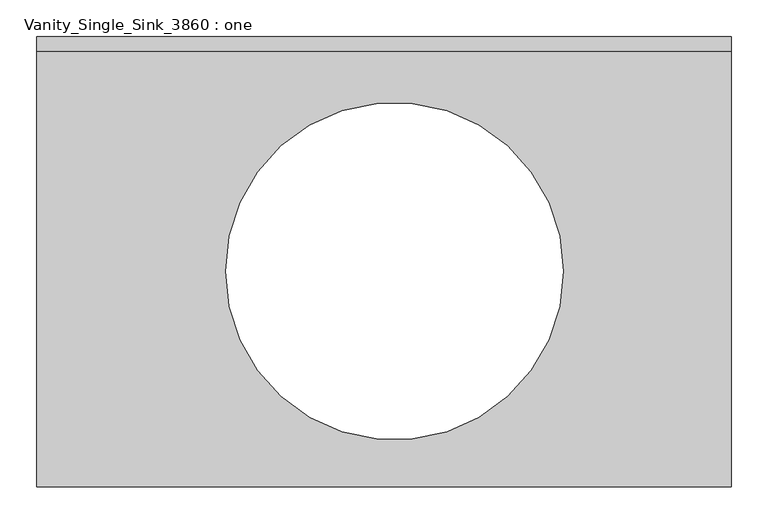
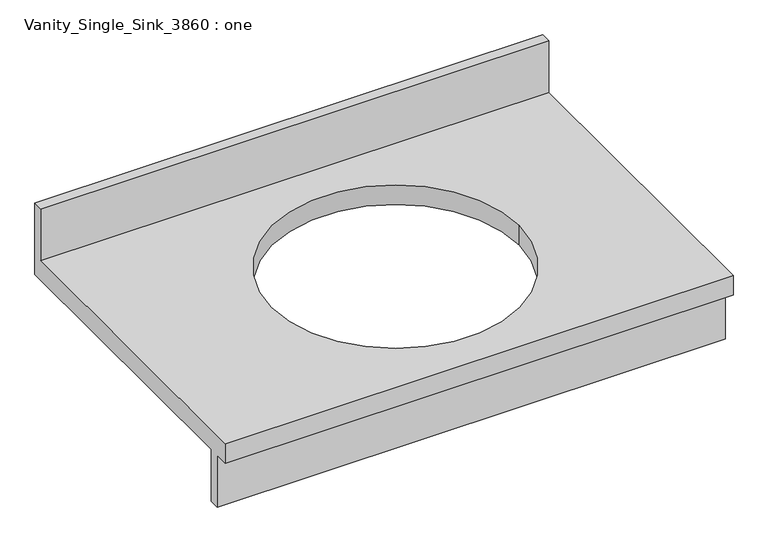
"""IFC4 building model written with IfcOpenShell, lengths in millimetres: furniture geometry, Vanity_Single_Sink_3860 : one."""

import ifcopenshell
import ifcopenshell.guid

model = None  # the IFC model being written
_history = None  # IfcOwnerHistory: only IFC2X3 demands one
_inside = {}  # id of a spatial element -> (the spatial element, [elements in it])
_under = {}  # id of a project, library or spatial element -> (it, [spatial elements below it])
_declared = {}  # id of a project -> (the project, [libraries it declares])
_typed = {}  # id of a type object -> (the type object, [elements of that type])
_made_of = {}  # id of a material, layer set ... -> (it, [elements and type objects made of it])


def new_model(schema):
    """Start an empty IFC model of exactly this schema.

    Asked for "IFC4X3", IfcOpenShell would pick the latest addendum, in which some entities
    have other attributes; the version numbers below select the first issue.
    IFC2X3 requires an IfcOwnerHistory on every rooted entity: one is made here for all.
    """
    global model, _history
    if schema == "IFC4X3":
        model = ifcopenshell.file(schema_version=(4, 3, 0, 0))
    else:
        model = ifcopenshell.file(schema=schema)
    _inside.clear()
    _under.clear()
    _declared.clear()
    _typed.clear()
    _made_of.clear()
    _history = None
    if model.schema == "IFC2X3":
        org = make("IfcOrganization", Name="unknown")
        user = make(
            "IfcPersonAndOrganization",
            ThePerson=make("IfcPerson", FamilyName="unknown"),
            TheOrganization=org,
        )
        app = make(
            "IfcApplication",
            ApplicationDeveloper=org,
            Version="unknown",
            ApplicationFullName="unknown",
            ApplicationIdentifier="unknown",
        )
        _history = make(
            "IfcOwnerHistory",
            OwningUser=user,
            OwningApplication=app,
            ChangeAction="ADDED",
            CreationDate=0,
        )
    return model


def make(cls, **values):
    """One entity of the class cls with the attributes given. An attribute that is None is left unset."""
    return model.create_entity(
        cls, **{name: value for name, value in values.items() if value is not None}
    )


def rooted(cls, **values):
    """An entity with a GlobalId (a new one), such as an element, a storey or a relation."""
    return make(cls, GlobalId=ifcopenshell.guid.new(), OwnerHistory=_history, **values)


def si_unit(unit_type, name, prefix=None):
    """IfcSIUnit, for example si_unit("LENGTHUNIT", "METRE", prefix="MILLI")."""
    return make("IfcSIUnit", UnitType=unit_type, Prefix=prefix, Name=name)


def assignment(units):
    """IfcUnitAssignment: the units of a project."""
    return None if units is None else make("IfcUnitAssignment", Units=units)


def point(xyz):
    """IfcCartesianPoint."""
    return None if xyz is None else make("IfcCartesianPoint", Coordinates=xyz)


def direction(xyz):
    """IfcDirection."""
    return None if xyz is None else make("IfcDirection", DirectionRatios=xyz)


def frame(location, z_axis=None, x_axis=None):
    """IfcAxis2Placement3D, a coordinate frame: its origin and axes. An axis left out is left unset."""
    return make(
        "IfcAxis2Placement3D",
        Location=point(location),
        Axis=direction(z_axis),
        RefDirection=direction(x_axis),
    )


def origin():
    """The frame at (0, 0, 0) with its axes left unset."""
    return frame((0.0, 0.0, 0.0))


def place(relative_to, where):
    """IfcLocalPlacement: puts the frame where relative to a parent placement (None: the world)."""
    return make(
        "IfcLocalPlacement", PlacementRelTo=relative_to, RelativePlacement=where
    )


def context(
    kind, dimensions, precision=None, world=None, true_north=None, identifier=None
):
    """IfcGeometricRepresentationContext, for example the 3D "Model" context."""
    return make(
        "IfcGeometricRepresentationContext",
        ContextIdentifier=identifier,
        ContextType=kind,
        CoordinateSpaceDimension=dimensions,
        Precision=precision,
        WorldCoordinateSystem=world,
        TrueNorth=true_north,
    )


def project(units=None, contexts=None):
    """IfcProject with its units and contexts."""
    return rooted(
        "IfcProject",
        Name="project",
        RepresentationContexts=contexts,
        UnitsInContext=assignment(units),
    )


def spatial(cls, under=None, at=None, **own):
    """A site, building, storey or space (cls), placed at a placement, below another one or the project."""
    s = rooted(cls, ObjectPlacement=at, **own)
    if under is not None:
        _under.setdefault(under.id(), (under, []))[1].append(s)
    return s


def polyline(points):
    """IfcPolyline through the points."""
    return make("IfcPolyline", Points=[point(p) for p in points])


def circle_curve(where, radius):
    """IfcCircle in the frame where."""
    return make("IfcCircle", Position=where, Radius=radius)


def shape(context_of_items, identifier, shape_type, items):
    """IfcShapeRepresentation: the items that make up one representation, for example the "Body"."""
    return make(
        "IfcShapeRepresentation",
        ContextOfItems=context_of_items,
        RepresentationIdentifier=identifier,
        RepresentationType=shape_type,
        Items=items,
    )


def source(mapping_origin, context_of_items, identifier, shape_type, items):
    """IfcRepresentationMap: a shape defined once, which mapped items show again and again."""
    return make(
        "IfcRepresentationMap",
        MappingOrigin=mapping_origin,
        MappedRepresentation=shape(context_of_items, identifier, shape_type, items),
    )


def transform(
    local_origin,
    x_axis=None,
    y_axis=None,
    z_axis=None,
    scale=None,
    scale2=None,
    scale3=None,
    uniform=True,
):
    """IfcCartesianTransformationOperator3D, or its non-uniform kind. x_axis, y_axis, z_axis: its Axis1, 2, 3."""
    if uniform:
        return make(
            "IfcCartesianTransformationOperator3D",
            Axis1=direction(x_axis),
            Axis2=direction(y_axis),
            LocalOrigin=point(local_origin),
            Scale=scale,
            Axis3=direction(z_axis),
        )
    return make(
        "IfcCartesianTransformationOperator3DnonUniform",
        Axis1=direction(x_axis),
        Axis2=direction(y_axis),
        LocalOrigin=point(local_origin),
        Scale=scale,
        Axis3=direction(z_axis),
        Scale2=scale2,
        Scale3=scale3,
    )


def mapped(mapping_source, mapping_target):
    """IfcMappedItem: shows the shape of a source again, moved by a transform."""
    return make(
        "IfcMappedItem", MappingSource=mapping_source, MappingTarget=mapping_target
    )


def made_of(thing, what):
    """Note that an element or type object is made of a material, layer set ...; save() writes the relation."""
    if what is not None:
        _made_of.setdefault(what.id(), (what, []))[1].append(thing)
    return thing


def element(
    cls,
    number,
    at=None,
    inside=None,
    cuts=None,
    type_object=None,
    material=None,
    context=None,
    identifier="Body",
    shape_type=None,
    held_by="IfcProductDefinitionShape",
    body=None,
    shapes=None,
    **own,
):
    """One element of the class cls, such as IfcWall. Its Tag is "e" and its number.

    at: its placement. inside: the storey or other place that contains it. cuts: it is an
    opening in that element (IfcRelVoidsElement). A single representation is given by context,
    identifier, shape_type and body (its items); several are given by shapes. held_by: the class
    of the entity that holds the representations. save() writes the other relations.
    """
    e = rooted(cls, Tag="e%d" % number, ObjectPlacement=at, **own)
    if body is not None:
        shapes = [shape(context, identifier, shape_type, body)]
    if shapes is not None:
        e.Representation = make(held_by, Representations=shapes)
    if inside is not None:
        _inside.setdefault(inside.id(), (inside, []))[1].append(e)
    if cuts is not None:
        rooted(
            "IfcRelVoidsElement", RelatingBuildingElement=cuts, RelatedOpeningElement=e
        )
    if type_object is not None:
        _typed.setdefault(type_object.id(), (type_object, []))[1].append(e)
    return made_of(e, material)


def aggregate(whole, parts):
    """IfcRelAggregates: a whole, such as a stair, and the parts it consists of."""
    return rooted("IfcRelAggregates", RelatingObject=whole, RelatedObjects=parts)


def save(model, path):
    """Write the relations noted so far, then the file.

    IfcRelAggregates (storeys below a building ...), IfcRelContainedInSpatialStructure (elements
    in a storey), IfcRelDefinesByType, IfcRelAssociatesMaterial and IfcRelDeclares: one each for
    every whole, place, type object, material and project.
    """
    for whole, parts in _under.values():
        aggregate(whole, parts)
    for where, things in _inside.values():
        rooted(
            "IfcRelContainedInSpatialStructure",
            RelatedElements=things,
            RelatingStructure=where,
        )
    for kind, things in _typed.values():
        rooted("IfcRelDefinesByType", RelatedObjects=things, RelatingType=kind)
    for what, things in _made_of.values():
        rooted("IfcRelAssociatesMaterial", RelatedObjects=things, RelatingMaterial=what)
    for by, libraries in _declared.values():
        rooted("IfcRelDeclares", RelatingContext=by, RelatedDefinitions=libraries)
    model.write(path)


def plane_surface(at):
    """IfcPlane: the flat surface through the origin of the frame at, square to its z axis."""
    return make("IfcPlane", Position=at)


def revolved_surface(curve, axis_point, axis_direction):
    """IfcSurfaceOfRevolution: the curve turned about the line through axis_point along axis_direction."""
    return make(
        "IfcSurfaceOfRevolution",
        SweptCurve=make("IfcArbitraryOpenProfileDef", ProfileType="CURVE", Curve=curve),
        AxisPosition=make("IfcAxis1Placement", Location=point(axis_point), Axis=direction(axis_direction)),
    )


def advanced_brep(points, edges, surfaces, faces):
    """IfcAdvancedBrep: a solid bounded by faces that lie on surfaces and meet in shared edges.

    An edge is (start, end): straight between two places in points (the first is 0);
    or (start, end, curve); or (start, end, curve, False) where it runs against its curve.
    A face is (place in surfaces, loops), or (place, loops, False) where it looks against
    its surface's normal. A loop lists edges by number (the first is 1), with a minus sign
    where the edge is run from its end to its start. The first loop is the outer one.
    """
    corners = [point(p) for p in points]
    vertices = [make("IfcVertexPoint", VertexGeometry=c) for c in corners]
    made = []
    for start, end, *more in edges:
        made.append(
            make(
                "IfcEdgeCurve",
                EdgeStart=vertices[start],
                EdgeEnd=vertices[end],
                EdgeGeometry=more[0] if more else make("IfcPolyline", Points=[corners[start], corners[end]]),
                SameSense=more[1] if len(more) > 1 else True,
            )
        )
    hull = []
    for where, loops, *sense in faces:
        bounds = []
        for j, loop in enumerate(loops):
            ring = [make("IfcOrientedEdge", EdgeElement=made[abs(k) - 1], Orientation=k > 0) for k in loop]
            bounds.append(
                make(
                    "IfcFaceOuterBound" if j == 0 else "IfcFaceBound",
                    Bound=make("IfcEdgeLoop", EdgeList=ring),
                    Orientation=True,
                )
            )
        hull.append(make("IfcAdvancedFace", Bounds=bounds, FaceSurface=surfaces[where], SameSense=sense[0] if sense else True))
    return make("IfcAdvancedBrep", Outer=make("IfcClosedShell", CfsFaces=hull))


def vanity_single_sink_3860_one_22dd408e(model_context):
    return source(origin(), model_context, "Body", "AdvancedBrep", [
        advanced_brep(
        [(-1327.4622951, -609.6, 863.6), (-387.6622951, -609.6, 863.6), (-387.6622951, -19.05, 863.6), (-1327.4622951, -19.05, 863.6), (-614.9287925, -317.5, 863.6), (-1072.1287925, -317.5, 863.6), (-387.6622951, -609.6, 825.5), (-1327.4622951, -609.6, 825.5), (-1327.4622951, -584.2, 825.5), (-387.6622951, -584.2, 825.5), (-1327.4622951, 0.0, 825.5), (-387.6622951, 0.0, 825.5), (-387.6622951, -565.15, 825.5), (-1327.4622951, -565.15, 825.5), (-1072.1287925, -317.5, 825.5), (-614.9287925, -317.5, 825.5), (-1327.4622951, 0.0, 965.2), (-387.6622951, 0.0, 965.2), (-1327.4622951, -19.05, 965.2), (-1327.4622951, -565.15, 723.9), (-1327.4622951, -584.2, 723.9), (-387.6622951, -584.2, 723.9), (-387.6622951, -565.15, 723.9), (-387.6622951, -19.05, 965.2)],
        [
            (0, 1),
            (1, 2),
            (2, 3),
            (3, 0),
            (4, 5, circle_curve(frame((-843.5287925, -317.5, 863.6), z_axis=(0.0, 0.0, -1.0), x_axis=(1.0, 0.0, 0.0)), 228.6)),
            (5, 4, circle_curve(frame((-843.5287925, -317.5, 863.6), z_axis=(0.0, 0.0, -1.0), x_axis=(1.0, 0.0, 0.0)), 228.6)),
            (6, 7),
            (7, 8),
            (8, 9),
            (9, 6),
            (10, 11),
            (11, 12),
            (12, 13),
            (13, 10),
            (14, 15, circle_curve(frame((-843.5287925, -317.5, 825.5), z_axis=(0.0, 0.0, 1.0), x_axis=(1.0, 0.0, 0.0)), 228.6)),
            (15, 14, circle_curve(frame((-843.5287925, -317.5, 825.5), z_axis=(0.0, 0.0, 1.0), x_axis=(1.0, 0.0, 0.0)), 228.6)),
            (10, 16),
            (16, 17),
            (17, 11),
            (7, 0),
            (3, 18),
            (18, 16),
            (13, 19),
            (19, 20),
            (20, 8),
            (6, 1),
            (9, 21),
            (21, 22),
            (22, 12),
            (17, 23),
            (23, 2),
            (18, 23),
            (4, 15),
            (14, 5),
            (21, 20),
            (19, 22),
        ],
        [
            plane_surface(frame((-1327.4622951, 0.0, 863.6), z_axis=(0.0, 0.0, 1.0), x_axis=(-1.0, 0.0, 0.0))),
            plane_surface(frame((-1327.4622951, 0.0, 825.5), z_axis=(0.0, 0.0, -1.0), x_axis=(1.0, 0.0, 0.0))),
            plane_surface(frame((-387.6622951, 0.0, 863.6), z_axis=(0.0, 1.0, 0.0), x_axis=(0.0, 0.0, -1.0))),
            plane_surface(frame((-1327.4622951, 0.0, 863.6), z_axis=(-1.0, 0.0, 0.0), x_axis=(0.0, 0.0, -1.0))),
            plane_surface(frame((-1327.4622951, -609.6, 863.6), z_axis=(0.0, -1.0, 0.0), x_axis=(0.0, 0.0, -1.0))),
            plane_surface(frame((-387.6622951, -609.6, 863.6), z_axis=(1.0, 0.0, 0.0), x_axis=(0.0, 0.0, -1.0))),
            plane_surface(frame((-1327.4622951, 0.0, 965.2), z_axis=(0.0, 0.0, 1.0), x_axis=(0.0, -1.0, 0.0))),
            plane_surface(frame((-1327.4622951, -19.05, 965.2), z_axis=(0.0, -1.0, 0.0), x_axis=(0.0, 0.0, -1.0))),
            revolved_surface(polyline([(-614.9287925, -317.5, 863.6), (-614.9287925, -317.5, 825.5)]), (-843.5287925, -317.5, 825.5), (0.0, 0.0, 1.0)),
            plane_surface(frame((-1327.4622951, -565.15, 723.9), z_axis=(0.0, 0.0, -1.0), x_axis=(1.0, 0.0, 0.0))),
            plane_surface(frame((-387.6622951, -565.15, 825.5), z_axis=(0.0, 1.0, 0.0), x_axis=(0.0, 0.0, -1.0))),
            plane_surface(frame((-1327.4622951, -584.2, 825.5), z_axis=(0.0, -1.0, 0.0), x_axis=(0.0, 0.0, -1.0))),
        ],
        [
            (0, [[1, 2, 3, 4], [5, 6]]),
            (1, [[7, 8, 9, 10]]),
            (1, [[11, 12, 13, 14], [15, 16]]),
            (2, [[-11, 17, 18, 19]]),
            (3, [[20, -4, 21, 22, -17, -14, 23, 24, 25, -8]]),
            (4, [[-1, -20, -7, 26]]),
            (5, [[-26, -10, 27, 28, 29, -12, -19, 30, 31, -2]]),
            (6, [[-22, 32, -30, -18]]),
            (7, [[-32, -21, -3, -31]]),
            (8, [[33, -15, 34, -5]]),
            (8, [[-33, -6, -34, -16]]),
            (9, [[-28, 35, -24, 36]]),
            (10, [[-36, -23, -13, -29]]),
            (11, [[-35, -27, -9, -25]]),
        ],
    ),
    ])


if __name__ == "__main__":
    model = new_model("IFC4")
    model_context = context("Model", 3, world=origin())
    ifc_project = project(units=[si_unit("LENGTHUNIT", "METRE", prefix="MILLI")], contexts=[model_context])
    site = spatial("IfcSite", under=ifc_project)
    building = spatial("IfcBuilding", under=site)
    placement = place(None, origin())
    vanity_single_sink_3860_one_shape = vanity_single_sink_3860_one_22dd408e(model_context)
    element("IfcFurniture", 1, ObjectType="Vanity_Single_Sink_3860 : one", at=placement, inside=building, context=model_context, shape_type="MappedRepresentation", body=[
        mapped(vanity_single_sink_3860_one_shape, transform((0.0, 0.0, 0.0), x_axis=(1.0, 0.0, 0.0), y_axis=(0.0, 1.0, 0.0), z_axis=(0.0, 0.0, 1.0))),
    ])
    save(model, "model.ifc")

# Revit data of these elements
# Type "Vanity_Single_Sink_3860 : one"
#   Assembly Code = "C1030400"
#   Counter Thickness = 0' - 1 1/2"
#   Depth = 2' - 0"
#   Height = 2' - 10"
#   Length [instance default] = 4' - 0"
#   Sink Location Left [instance default] = 2' - 0"
#   Sink to Back Wall = 0' - 4"
#   Sink Opening Width [instance default] = 1' - 5"
#   Counter Top = Casework - Vanity Top
#   Width = 0
# Element 1 (IfcFurniture, "Vanity_Single_Sink_3860 : one")
#   Length = 3' - 1"
#   Sink Location Left = 1' - 7.0525"
#   Materials on its faces: "Casework - Vanity Top"
# Materials
#   "Casework - Vanity Top": class "Unassigned", colour RGB 210 200 171, transparency 0, Comments = "Rendering appearance not upgraded "
